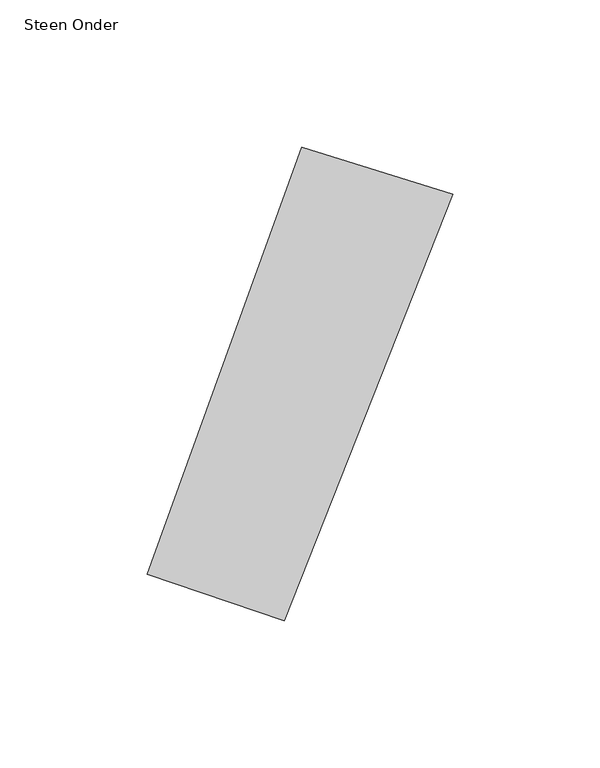
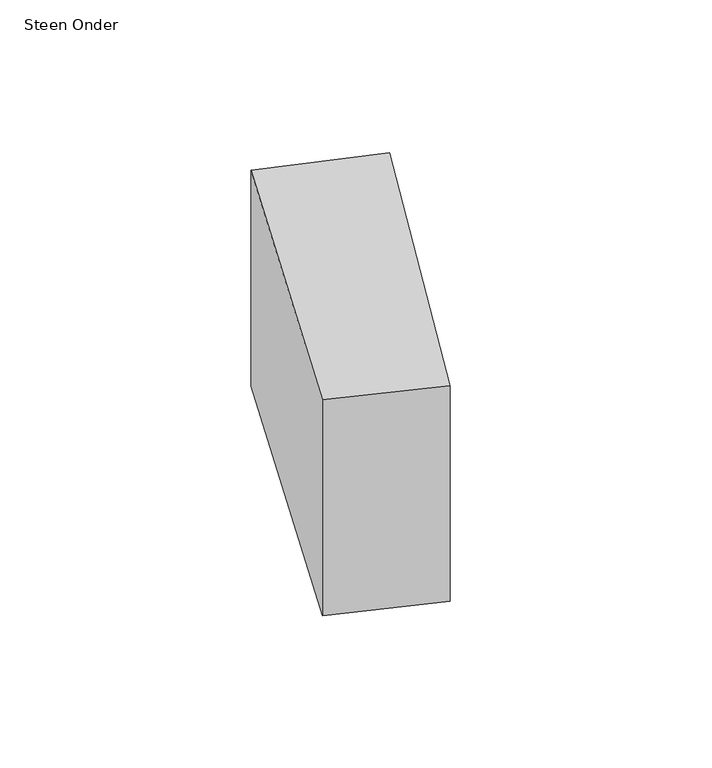
"""IFC4 building model written with IfcOpenShell, lengths in millimetres: proxy geometry, 00_GMA_steen_versie_4 : Steen Onder."""

from ifc_helpers import new_model, si_unit, origin, origin_with_axes, place, context, project, spatial, polyline, outline, extrude, source, transform, mapped, element, save


def steen_onder_141eb73a(model_context):
    return source(origin(), model_context, "Body", "SweptSolid", [
        extrude(outline(polyline([(128.5689911, 140.4928828), (71.2811692, -4.603009), (24.6281455, 11.3152916), (77.1603575, 156.542947), (128.5689911, 140.4928828)])), origin_with_axes(), (0.0, 0.0, 1.0), 100.0),
    ])


if __name__ == "__main__":
    model = new_model("IFC4")
    model_context = context("Model", 3, world=origin())
    ifc_project = project(units=[si_unit("LENGTHUNIT", "METRE", prefix="MILLI")], contexts=[model_context])
    site = spatial("IfcSite", under=ifc_project)
    building = spatial("IfcBuilding", under=site)
    placement = place(None, origin())
    steen_onder_shape = steen_onder_141eb73a(model_context)
    element("IfcBuildingElementProxy", 1, Name="00_GMA_steen_versie_4 : Steen Onder", ObjectType="00_GMA_steen_versie_4 : Steen Onder", at=placement, inside=building, context=model_context, shape_type="MappedRepresentation", body=[
        mapped(steen_onder_shape, transform((0.0, 0.0, 0.0), x_axis=(1.0, 0.0, 0.0), y_axis=(0.0, 1.0, 0.0), z_axis=(0.0, 0.0, 1.0))),
    ])
    save(model, "model.ifc")

# Revit data of these elements
# Type "00_GMA_steen_versie_4 : Steen Onder"
#   StootVoegHalfBoven [instance default] = 5 mm
#   StootVoegHalf [instance default] = 5 mm
#   StootVoegBreedteOnder = 10 mm
#   StootVoegBreedteBoven = 10 mm
#   Steendikte = 100 mm
#   LintVoegOnderHalf = 0 mm
#   LintVoegOnder = 0 mm
#   LintVoegBovenHalf = 5 mm
#   LintVoegBoven = 10 mm
#   materiaal = none
#   MateriaalVoeg = none
#   Default Elevation = 0
